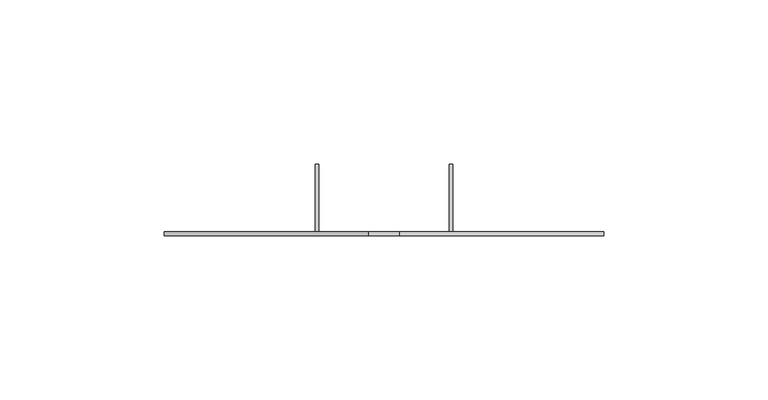
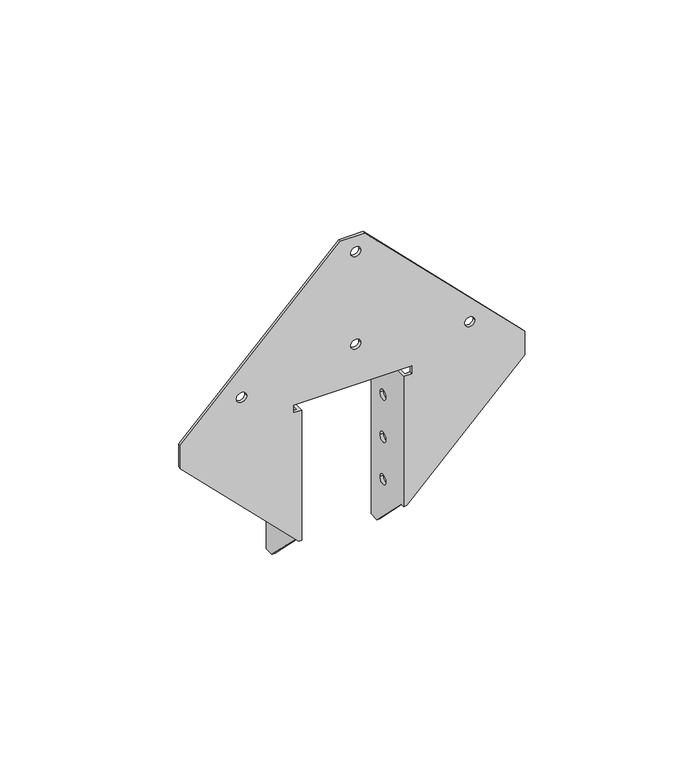
"""IFC4 building model written with IfcOpenShell, lengths in millimetres: proxy geometry, Simpson Strong-Tie H1 : Simpson Strong-Tie H1."""

from ifc_helpers import new_model, si_unit, frame, origin, place, context, project, spatial, polyline, circle_curve, source, transform, mapped, element, save
from ifc_brep_helpers import plane_surface, revolved_surface, advanced_brep


def generic_models_343c88cb(model_context):
    return source(origin(), model_context, "Body", "AdvancedBrep", [
        advanced_brep(
        [(-0.790575, 0.0, 54.76875), (3.171825, 0.0, 54.76875), (3.171825, 1.18872, 54.76875), (-0.790575, 1.18872, 54.76875), (-0.790575, 0.0, 16.66875), (3.171825, 0.0, 16.66875), (3.171825, 1.18872, 16.66875), (-0.790575, 1.18872, 16.66875), (43.659425, 0.0, 10.31875), (47.621825, 0.0, 10.31875), (47.621825, 1.18872, 10.31875), (43.659425, 1.18872, 10.31875), (-45.240575, 0.0, 10.31875), (-41.278175, 0.0, 10.31875), (-41.278175, 1.18872, 10.31875), (-45.240575, 1.18872, 10.31875), (19.84756, 11.902103, -19.05), (19.84756, 15.864503, -19.05), (21.03628, 15.864503, -19.05), (21.03628, 11.902103, -19.05), (19.84756, 11.902103, -36.5125), (19.84756, 15.864503, -36.5125), (21.03628, 15.864503, -36.5125), (21.03628, 11.902103, -36.5125), (19.84756, 11.902103, -53.975), (19.84756, 15.864503, -53.975), (21.03628, 15.864503, -53.975), (21.03628, 11.902103, -53.975), (-21.03628, 11.902103, -57.15), (-21.03628, 15.864503, -57.15), (-19.84756, 15.864503, -57.15), (-19.84756, 11.902103, -57.15), (-21.03628, 11.902103, -39.6875), (-21.03628, 15.864503, -39.6875), (-19.84756, 15.864503, -39.6875), (-19.84756, 11.902103, -39.6875), (-21.03628, 11.902103, -22.225), (-21.03628, 15.864503, -22.225), (-19.84756, 15.864503, -22.225), (-19.84756, 11.902103, -22.225), (23.08225, 0.0, 0.0), (23.08225, 1.18872, 0.0), (23.08225, 1.18872, -3.175), (23.08225, 0.0, -3.175), (21.03628, 0.0, -56.758894), (19.84756, 0.0, -56.758894), (19.84756, 1.698923, -56.758894), (21.03628, 1.698923, -56.758894), (21.03628, 1.18872, -56.758894), (19.84756, 0.0, -3.175), (21.03628, 1.18872, -3.175), (21.03628, 21.820803, -3.175), (19.84756, 21.820803, -3.175), (-23.08225, 1.18872, 0.0), (-23.08225, 1.18872, -3.175), (-21.03628, 1.18872, -3.175), (-21.03628, 1.18872, -56.758894), (-67.071875, 1.18872, -10.723299), (-67.071875, 1.18872, -1.182951), (-4.770174, 1.18872, 61.11875), (4.770174, 1.18872, 61.11875), (67.071875, 1.18872, -1.182951), (67.071875, 1.18872, -10.723299), (19.84756, 21.820803, -73.025), (19.84756, 17.965029, -73.025), (-21.03628, 1.698923, -56.758894), (-19.84756, 1.698923, -56.758894), (-19.84756, 0.0, -56.758894), (-21.03628, 0.0, -56.758894), (67.071875, 0.0, -10.723299), (67.071875, 0.0, -1.182951), (4.770174, 0.0, 61.11875), (-4.770174, 0.0, 61.11875), (-67.071875, 0.0, -1.182951), (-67.071875, 0.0, -10.723299), (-19.84756, 0.0, -3.175), (-23.08225, 0.0, -3.175), (-23.08225, 0.0, 0.0), (-19.84756, 21.820803, -3.175), (-21.03628, 21.820803, -3.175), (21.03628, 17.965029, -73.025), (21.03628, 21.820803, -73.025), (-19.84756, 17.965029, -73.025), (-19.84756, 21.820803, -73.025), (-21.03628, 21.820803, -73.025), (-21.03628, 17.965029, -73.025)],
        [
            (0, 1, circle_curve(frame((1.190625, 0.0, 54.76875), z_axis=(0.0, -1.0, 0.0), x_axis=(-1.0, 0.0, 0.0)), 1.9812)),
            (1, 2),
            (2, 3, circle_curve(frame((1.190625, 1.18872, 54.76875), z_axis=(0.0, 1.0, 0.0), x_axis=(-1.0, 0.0, 0.0)), 1.9812)),
            (3, 0),
            (4, 5, circle_curve(frame((1.190625, 0.0, 16.66875), z_axis=(0.0, -1.0, 0.0), x_axis=(-1.0, 0.0, 0.0)), 1.9812)),
            (5, 6),
            (6, 7, circle_curve(frame((1.190625, 1.18872, 16.66875), z_axis=(0.0, 1.0, 0.0), x_axis=(-1.0, 0.0, 0.0)), 1.9812)),
            (7, 4),
            (8, 9, circle_curve(frame((45.640625, 0.0, 10.31875), z_axis=(0.0, -1.0, 0.0), x_axis=(-1.0, 0.0, 0.0)), 1.9812)),
            (9, 10),
            (10, 11, circle_curve(frame((45.640625, 1.18872, 10.31875), z_axis=(0.0, 1.0, 0.0), x_axis=(-1.0, 0.0, 0.0)), 1.9812)),
            (11, 8),
            (12, 13, circle_curve(frame((-43.259375, 0.0, 10.31875), z_axis=(0.0, -1.0, 0.0), x_axis=(-1.0, 0.0, 0.0)), 1.9812)),
            (13, 14),
            (14, 15, circle_curve(frame((-43.259375, 1.18872, 10.31875), z_axis=(0.0, 1.0, 0.0), x_axis=(-1.0, 0.0, 0.0)), 1.9812)),
            (15, 12),
            (16, 17, circle_curve(frame((19.84756, 13.883303, -19.05), z_axis=(-1.0, 0.0, 0.0), x_axis=(0.0, -1.0, 0.0)), 1.9812)),
            (17, 18),
            (18, 19, circle_curve(frame((21.03628, 13.883303, -19.05), z_axis=(1.0, 0.0, 0.0), x_axis=(0.0, -1.0, 0.0)), 1.9812)),
            (19, 16),
            (20, 21, circle_curve(frame((19.84756, 13.883303, -36.5125), z_axis=(-1.0, 0.0, 0.0), x_axis=(0.0, -1.0, 0.0)), 1.9812)),
            (21, 22),
            (22, 23, circle_curve(frame((21.03628, 13.883303, -36.5125), z_axis=(1.0, 0.0, 0.0), x_axis=(0.0, -1.0, 0.0)), 1.9812)),
            (23, 20),
            (24, 25, circle_curve(frame((19.84756, 13.883303, -53.975), z_axis=(-1.0, 0.0, 0.0), x_axis=(0.0, -1.0, 0.0)), 1.9812)),
            (25, 26),
            (26, 27, circle_curve(frame((21.03628, 13.883303, -53.975), z_axis=(1.0, 0.0, 0.0), x_axis=(0.0, -1.0, 0.0)), 1.9812)),
            (27, 24),
            (28, 29, circle_curve(frame((-21.03628, 13.883303, -57.15), z_axis=(-1.0, 0.0, 0.0), x_axis=(0.0, -1.0, 0.0)), 1.9812)),
            (29, 30),
            (30, 31, circle_curve(frame((-19.84756, 13.883303, -57.15), z_axis=(1.0, 0.0, 0.0), x_axis=(0.0, -1.0, 0.0)), 1.9812)),
            (31, 28),
            (32, 33, circle_curve(frame((-21.03628, 13.883303, -39.6875), z_axis=(-1.0, 0.0, 0.0), x_axis=(0.0, -1.0, 0.0)), 1.9812)),
            (33, 34),
            (34, 35, circle_curve(frame((-19.84756, 13.883303, -39.6875), z_axis=(1.0, 0.0, 0.0), x_axis=(0.0, -1.0, 0.0)), 1.9812)),
            (35, 32),
            (36, 37, circle_curve(frame((-21.03628, 13.883303, -22.225), z_axis=(-1.0, 0.0, 0.0), x_axis=(0.0, -1.0, 0.0)), 1.9812)),
            (37, 38),
            (38, 39, circle_curve(frame((-19.84756, 13.883303, -22.225), z_axis=(1.0, 0.0, 0.0), x_axis=(0.0, -1.0, 0.0)), 1.9812)),
            (39, 36),
            (40, 41),
            (41, 42),
            (42, 43),
            (43, 40),
            (44, 45),
            (45, 46),
            (46, 47),
            (47, 48),
            (48, 44),
            (49, 43),
            (42, 50),
            (50, 51),
            (51, 52),
            (52, 49),
            (53, 54),
            (54, 55),
            (55, 56),
            (56, 57),
            (57, 58),
            (58, 59),
            (59, 60),
            (60, 61),
            (61, 62),
            (62, 48),
            (48, 50),
            (41, 53),
            (14, 15, circle_curve(frame((-43.259375, 1.18872, 10.31875), z_axis=(0.0, -1.0, 0.0), x_axis=(-1.0, 0.0, 0.0)), 1.9812)),
            (10, 11, circle_curve(frame((45.640625, 1.18872, 10.31875), z_axis=(0.0, -1.0, 0.0), x_axis=(-1.0, 0.0, 0.0)), 1.9812)),
            (6, 7, circle_curve(frame((1.190625, 1.18872, 16.66875), z_axis=(0.0, -1.0, 0.0), x_axis=(-1.0, 0.0, 0.0)), 1.9812)),
            (2, 3, circle_curve(frame((1.190625, 1.18872, 54.76875), z_axis=(0.0, -1.0, 0.0), x_axis=(-1.0, 0.0, 0.0)), 1.9812)),
            (45, 49),
            (52, 63),
            (63, 64),
            (64, 46),
            (16, 17, circle_curve(frame((19.84756, 13.883303, -19.05), z_axis=(1.0, 0.0, 0.0), x_axis=(0.0, -1.0, 0.0)), 1.9812)),
            (20, 21, circle_curve(frame((19.84756, 13.883303, -36.5125), z_axis=(1.0, 0.0, 0.0), x_axis=(0.0, -1.0, 0.0)), 1.9812)),
            (24, 25, circle_curve(frame((19.84756, 13.883303, -53.975), z_axis=(1.0, 0.0, 0.0), x_axis=(0.0, -1.0, 0.0)), 1.9812)),
            (56, 65),
            (65, 66),
            (66, 67),
            (67, 68),
            (68, 56),
            (44, 69),
            (69, 70),
            (70, 71),
            (71, 72),
            (72, 73),
            (73, 74),
            (74, 68),
            (67, 75),
            (75, 76),
            (76, 77),
            (77, 40),
            (0, 1, circle_curve(frame((1.190625, 0.0, 54.76875), z_axis=(0.0, 1.0, 0.0), x_axis=(-1.0, 0.0, 0.0)), 1.9812)),
            (4, 5, circle_curve(frame((1.190625, 0.0, 16.66875), z_axis=(0.0, 1.0, 0.0), x_axis=(-1.0, 0.0, 0.0)), 1.9812)),
            (8, 9, circle_curve(frame((45.640625, 0.0, 10.31875), z_axis=(0.0, 1.0, 0.0), x_axis=(-1.0, 0.0, 0.0)), 1.9812)),
            (12, 13, circle_curve(frame((-43.259375, 0.0, 10.31875), z_axis=(0.0, 1.0, 0.0), x_axis=(-1.0, 0.0, 0.0)), 1.9812)),
            (74, 57),
            (76, 54),
            (53, 77),
            (75, 78),
            (78, 79),
            (79, 55),
            (64, 80),
            (80, 47),
            (80, 81),
            (81, 51),
            (26, 27, circle_curve(frame((21.03628, 13.883303, -53.975), z_axis=(-1.0, 0.0, 0.0), x_axis=(0.0, -1.0, 0.0)), 1.9812)),
            (22, 23, circle_curve(frame((21.03628, 13.883303, -36.5125), z_axis=(-1.0, 0.0, 0.0), x_axis=(0.0, -1.0, 0.0)), 1.9812)),
            (18, 19, circle_curve(frame((21.03628, 13.883303, -19.05), z_axis=(-1.0, 0.0, 0.0), x_axis=(0.0, -1.0, 0.0)), 1.9812)),
            (66, 82),
            (82, 83),
            (83, 78),
            (38, 39, circle_curve(frame((-19.84756, 13.883303, -22.225), z_axis=(-1.0, 0.0, 0.0), x_axis=(0.0, -1.0, 0.0)), 1.9812)),
            (34, 35, circle_curve(frame((-19.84756, 13.883303, -39.6875), z_axis=(-1.0, 0.0, 0.0), x_axis=(0.0, -1.0, 0.0)), 1.9812)),
            (30, 31, circle_curve(frame((-19.84756, 13.883303, -57.15), z_axis=(-1.0, 0.0, 0.0), x_axis=(0.0, -1.0, 0.0)), 1.9812)),
            (79, 84),
            (84, 85),
            (85, 65),
            (28, 29, circle_curve(frame((-21.03628, 13.883303, -57.15), z_axis=(1.0, 0.0, 0.0), x_axis=(0.0, -1.0, 0.0)), 1.9812)),
            (32, 33, circle_curve(frame((-21.03628, 13.883303, -39.6875), z_axis=(1.0, 0.0, 0.0), x_axis=(0.0, -1.0, 0.0)), 1.9812)),
            (36, 37, circle_curve(frame((-21.03628, 13.883303, -22.225), z_axis=(1.0, 0.0, 0.0), x_axis=(0.0, -1.0, 0.0)), 1.9812)),
            (85, 82),
            (72, 59),
            (58, 73),
            (84, 83),
            (81, 63),
            (62, 69),
            (61, 70),
            (60, 71),
        ],
        [
            revolved_surface(polyline([(-0.790575, 0.0, 54.76875), (-0.790575, 1.18872, 54.76875)]), (1.190625, 1.18872, 54.76875), (0.0, -1.0, 0.0)),
            revolved_surface(polyline([(-0.790575, 0.0, 16.66875), (-0.790575, 1.18872, 16.66875)]), (1.190625, 1.18872, 16.66875), (0.0, -1.0, 0.0)),
            revolved_surface(polyline([(43.659425, 0.0, 10.31875), (43.659425, 1.18872, 10.31875)]), (45.640625, 1.18872, 10.31875), (0.0, -1.0, 0.0)),
            revolved_surface(polyline([(-45.240575, 0.0, 10.31875), (-45.240575, 1.18872, 10.31875)]), (-43.259375, 1.18872, 10.31875), (0.0, -1.0, 0.0)),
            revolved_surface(polyline([(19.84756, 11.902103, -19.05), (21.03628, 11.902103, -19.05)]), (21.03628, 13.883303, -19.05), (-1.0, 0.0, 0.0)),
            revolved_surface(polyline([(19.84756, 11.902103, -36.5125), (21.03628, 11.902103, -36.5125)]), (21.03628, 13.883303, -36.5125), (-1.0, 0.0, 0.0)),
            revolved_surface(polyline([(19.84756, 11.902103, -53.975), (21.03628, 11.902103, -53.975)]), (21.03628, 13.883303, -53.975), (-1.0, 0.0, 0.0)),
            revolved_surface(polyline([(-21.03628, 11.902103, -57.15), (-19.84756, 11.902103, -57.15)]), (-19.84756, 13.883303, -57.15), (-1.0, 0.0, 0.0)),
            revolved_surface(polyline([(-21.03628, 11.902103, -39.6875), (-19.84756, 11.902103, -39.6875)]), (-19.84756, 13.883303, -39.6875), (-1.0, 0.0, 0.0)),
            revolved_surface(polyline([(-21.03628, 11.902103, -22.225), (-19.84756, 11.902103, -22.225)]), (-19.84756, 13.883303, -22.225), (-1.0, 0.0, 0.0)),
            plane_surface(frame((23.08225, 1.18872, -3.175), z_axis=(-1.0, 0.0, 0.0), x_axis=(0.0, 0.0, 1.0))),
            plane_surface(frame((19.84756, 0.0, -56.758894), z_axis=(0.0, 0.0, -1.0), x_axis=(1.0, 0.0, 0.0))),
            plane_surface(frame((21.03628, 1.240453, -3.175), z_axis=(0.0, 0.0, 1.0), x_axis=(1.0, 0.0, 0.0))),
            plane_surface(frame((0.0, 1.18872, -12.3047323), z_axis=(0.0, 1.0, 0.0), x_axis=(1.0, 0.0, 0.0))),
            plane_surface(frame((19.84756, 22.735203, -12.3047323), z_axis=(-1.0, 0.0, 0.0), x_axis=(0.0, -1.0, 0.0))),
            plane_surface(frame((-19.84756, 0.0, -56.758894), z_axis=(0.0, 0.0, -1.0), x_axis=(-1.0, 0.0, 0.0))),
            plane_surface(frame((0.0, 0.0, -12.3047323), z_axis=(0.0, -1.0, 0.0), x_axis=(1.0, 0.0, 0.0))),
            plane_surface(frame((-67.071875, 1.18872, -10.723299), z_axis=(-0.7071067811865432, 0.0, -0.7071067811865518), x_axis=(0.0, -1.0, 0.0))),
            plane_surface(frame((-23.08225, 1.18872, -3.175), z_axis=(1.0, 0.0, 0.0), x_axis=(0.0, 0.0, 1.0))),
            plane_surface(frame((-21.03628, 21.820803, -3.175), z_axis=(0.0, 0.0, 1.0), x_axis=(-1.0, 0.0, 0.0))),
            plane_surface(frame((21.03628, 17.965029, -73.025), z_axis=(0.0, -0.7071067811865476, -0.7071067811865475), x_axis=(1.0, 0.0, 0.0))),
            plane_surface(frame((21.03628, 22.735203, -12.3047323), z_axis=(1.0, 0.0, 0.0), x_axis=(0.0, -1.0, 0.0))),
            plane_surface(frame((-19.84756, 22.735203, -12.3047323), z_axis=(1.0, 0.0, 0.0), x_axis=(0.0, 1.0, 0.0))),
            plane_surface(frame((-21.03628, 22.735203, -12.3047323), z_axis=(-1.0, 0.0, 0.0), x_axis=(0.0, 1.0, 0.0))),
            plane_surface(frame((-4.770174, 1.18872, 61.11875), z_axis=(-0.7071067811865518, 0.0, 0.7071067811865434), x_axis=(0.0, -1.0, 0.0))),
            plane_surface(frame((-67.071875, 1.18872, -1.182951), z_axis=(-1.0, 0.0, 0.0), x_axis=(0.0, -1.0, 0.0))),
            plane_surface(frame((-21.03628, 17.965029, -73.025), z_axis=(0.0, 0.0, -1.0), x_axis=(1.0, 0.0, 0.0))),
            plane_surface(frame((-21.03628, 21.820803, -73.025), z_axis=(0.0, 1.0, 0.0), x_axis=(-1.0, 0.0, 0.0))),
            plane_surface(frame((-21.49475, 1.18872, 0.0), z_axis=(0.0, 0.0, -1.0), x_axis=(0.0, -1.0, 0.0))),
            plane_surface(frame((21.03628, 21.820803, -3.175), z_axis=(0.0, 1.0, 0.0), x_axis=(-1.0, 0.0, 0.0))),
            plane_surface(frame((21.03628, 21.820803, -73.025), z_axis=(0.0, 0.0, -1.0), x_axis=(-1.0, 0.0, 0.0))),
            plane_surface(frame((4.770174, 1.18872, -73.025), z_axis=(0.7071067811865519, 0.0, -0.7071067811865431), x_axis=(0.0, 1.0, 0.0))),
            plane_surface(frame((67.071875, 1.18872, -10.723299), z_axis=(1.0, 0.0, 0.0), x_axis=(0.0, 1.0, 0.0))),
            plane_surface(frame((67.071875, 1.18872, -1.182951), z_axis=(0.707106781186543, 0.0, 0.707106781186552), x_axis=(0.0, 1.0, 0.0))),
            plane_surface(frame((4.770174, 1.18872, 61.11875), z_axis=(0.0, 0.0, 1.0), x_axis=(0.0, 1.0, 0.0))),
        ],
        [
            (0, [[1, 2, 3, 4]]),
            (1, [[5, 6, 7, 8]]),
            (2, [[9, 10, 11, 12]]),
            (3, [[13, 14, 15, 16]]),
            (4, [[17, 18, 19, 20]]),
            (5, [[21, 22, 23, 24]]),
            (6, [[25, 26, 27, 28]]),
            (7, [[29, 30, 31, 32]]),
            (8, [[33, 34, 35, 36]]),
            (9, [[37, 38, 39, 40]]),
            (10, [[41, 42, 43, 44]]),
            (11, [[45, 46, 47, 48, 49]]),
            (12, [[50, -43, 51, 52, 53, 54]]),
            (13, [[55, 56, 57, 58, 59, 60, 61, 62, 63, 64, 65, -51, -42, 66], [67, -15], [68, -11], [69, -7], [70, -3]]),
            (14, [[71, -54, 72, 73, 74, -46], [-17, 75], [-21, 76], [-25, 77]]),
            (15, [[78, 79, 80, 81, 82]]),
            (16, [[-44, -50, -71, -45, 83, 84, 85, 86, 87, 88, 89, -81, 90, 91, 92, 93], [-1, 94], [-5, 95], [-9, 96], [-13, 97]]),
            (17, [[-89, 98, -58, -82]]),
            (18, [[99, -55, 100, -92]]),
            (19, [[-56, -99, -91, 101, 102, 103]]),
            (20, [[-47, -74, 104, 105]]),
            (21, [[-48, -105, 106, 107, -52, -65], [108, -27], [109, -23], [110, -19]]),
            (22, [[111, 112, 113, -101, -90, -80], [114, -39], [115, -35], [116, -31]]),
            (23, [[-57, -103, 117, 118, 119, -78], [-29, 120], [-33, 121], [-37, 122]]),
            (9, [[-114, -38, -122, -40]]),
            (8, [[-115, -34, -121, -36]]),
            (7, [[-116, -30, -120, -32]]),
            (6, [[-108, -26, -77, -28]]),
            (5, [[-109, -22, -76, -24]]),
            (4, [[-110, -18, -75, -20]]),
            (20, [[-79, -119, 123, -111]]),
            (3, [[-67, -14, -97, -16]]),
            (2, [[-68, -10, -96, -12]]),
            (1, [[-69, -6, -95, -8]]),
            (0, [[-70, -2, -94, -4]]),
            (24, [[124, -60, 125, -87]]),
            (25, [[-125, -59, -98, -88]]),
            (26, [[-123, -118, 126, -112]]),
            (27, [[-126, -117, -102, -113]]),
            (28, [[-41, -93, -100, -66]]),
            (29, [[-53, -107, 127, -72]]),
            (30, [[-127, -106, -104, -73]]),
            (31, [[-64, 128, -83, -49]]),
            (32, [[-128, -63, 129, -84]]),
            (33, [[-129, -62, 130, -85]]),
            (34, [[-130, -61, -124, -86]]),
        ],
    ),
    ])


if __name__ == "__main__":
    model = new_model("IFC4")
    model_context = context("Model", 3, world=origin())
    ifc_project = project(units=[si_unit("LENGTHUNIT", "METRE", prefix="MILLI")], contexts=[model_context])
    site = spatial("IfcSite", under=ifc_project)
    building = spatial("IfcBuilding", under=site)
    placement = place(None, origin())
    generic_models_shape = generic_models_343c88cb(model_context)
    element("IfcBuildingElementProxy", 1, Name="Simpson Strong-Tie H1 : Simpson Strong-Tie H1", ObjectType="Simpson Strong-Tie H1 : Simpson Strong-Tie H1", at=placement, inside=building, context=model_context, shape_type="MappedRepresentation", body=[
        mapped(generic_models_shape, transform((0.0, 0.0, 0.0), x_axis=(1.0, 0.0, 0.0), y_axis=(0.0, 1.0, 0.0), z_axis=(0.0, 0.0, 1.0))),
    ])
    save(model, "model.ifc")

# Revit data of these elements
# Type "Simpson Strong-Tie H1 : Simpson Strong-Tie H1"
#   Default Elevation = 0
# Element 1 (IfcBuildingElementProxy, "Simpson Strong-Tie H1 : Simpson Strong-Tie H1")
#   Materials on its faces: "Material __RGBA_0.749_0.749_0.749_1.000"
# Materials
#   "Material __RGBA_0.749_0.749_0.749_1.000": class "SAT", colour RGB 191 191 191, transparency 0
